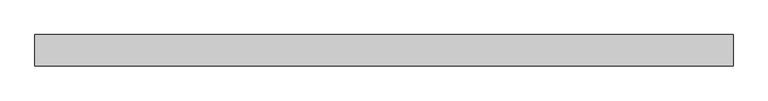
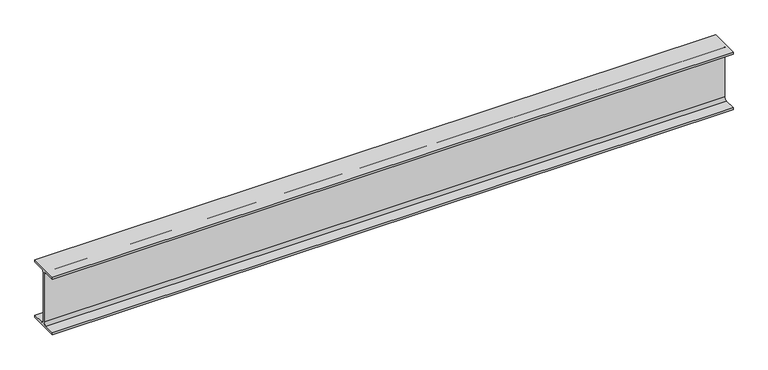
"""IFC4 building model written with IfcOpenShell, lengths in millimetres: beam geometry, 0912_Steel Framing_H-KSD3502 : H_SB_ASB_H-250x125x6x9."""

from ifc_helpers import new_model, si_unit, point, frame, frame_2d, origin, place, context, project, spatial, polyline, circle_curve, trimmed, segment, composite_curve, outline, extrude, source, transform, mapped, element, save


def beam_cbea06df(model_context):
    return source(origin(), model_context, "Body", "SweptSolid", [
        extrude(outline(composite_curve([segment(polyline([(62.5, -116.0), (62.5, -125.0), (-62.5, -125.0), (-62.5, -116.0), (-15.0, -116.0)]), True, "CONTINUOUS"), segment(trimmed(circle_curve(frame_2d((-15.0, -104.0)), 12.0), [point((-15.0, -116.0))], [point((-3.0, -104.0))], True, "CARTESIAN"), True, "CONTINUOUS"), segment(polyline([(-3.0, -104.0), (-3.0, 104.0)]), True, "CONTINUOUS"), segment(trimmed(circle_curve(frame_2d((-15.0, 104.0)), 12.0), [point((-3.0, 104.0))], [point((-15.0, 116.0))], True, "CARTESIAN"), True, "CONTINUOUS"), segment(polyline([(-15.0, 116.0), (-62.5, 116.0), (-62.5, 125.0), (62.5, 125.0), (62.5, 116.0), (15.0, 116.0)]), True, "CONTINUOUS"), segment(trimmed(circle_curve(frame_2d((15.0, 104.0)), 12.0), [point((15.0, 116.0))], [point((3.0, 104.0))], True, "CARTESIAN"), True, "CONTINUOUS"), segment(polyline([(3.0, 104.0), (3.0, -104.0)]), True, "CONTINUOUS"), segment(trimmed(circle_curve(frame_2d((15.0, -104.0)), 12.0), [point((3.0, -104.0))], [point((15.0, -116.0))], True, "CARTESIAN"), True, "CONTINUOUS"), segment(polyline([(15.0, -116.0), (62.5, -116.0)]), True, "CONTINUOUS")], self_intersect=False)), frame((-1382.2982577, 0.0, 0.0), z_axis=(1.0, 0.0, 0.0), x_axis=(0.0, 1.0, 0.0)), (0.0, 0.0, 1.0), 2794.5982507),
    ])


if __name__ == "__main__":
    model = new_model("IFC4")
    model_context = context("Model", 3, world=origin())
    ifc_project = project(units=[si_unit("LENGTHUNIT", "METRE", prefix="MILLI")], contexts=[model_context])
    site = spatial("IfcSite", under=ifc_project)
    building = spatial("IfcBuilding", under=site)
    placement = place(None, origin())
    beam_shape = beam_cbea06df(model_context)
    element("IfcBeam", 1, ObjectType="0912_Steel Framing_H-KSD3502 : H_SB_ASB_H-250x125x6x9", at=placement, inside=building, context=model_context, shape_type="MappedRepresentation", body=[
        mapped(beam_shape, transform((0.0, 0.0, 0.0), x_axis=(1.0, 0.0, 0.0), y_axis=(0.0, 1.0, 0.0), z_axis=(0.0, 0.0, 1.0))),
    ])
    save(model, "model.ifc")

# Revit data of these elements
# Type "0912_Steel Framing_H-KSD3502 : H_SB_ASB_H-250x125x6x9"
#   H_WM Code_1 = "S01AA003-00001 | Main Steel Structure Fabrication Work | Shelter/Building | Light Steel - Standard (30KG/M>Weight) | Material: (   )"
#   H_WM Code_2 = "S03AA029-00001 | Main Steel Structure Erection Work | Shelter/Building | Light Steel (30KG/M>Weight) | Material: (   )"
#   H_WM Code_3 = "S01AA010-00001 | Main Steel Structure Fabrication Work | Shelter/Building | Steel Painting/Coating | for Non-Fireproofed Steel Surface, Surface Preparation, Primer, Second & Final Coat | Material: (   )"
#   H_Q'ty Cal Type Tag = "SB-Q2"
#   Width = 12.5 cm
#   Web Thickness = 0.6 cm
#   Web Fillet = 1.2 cm
#   Warping Constant = 42539.8 cm⁶
#   W = 0
#   Torsional Moment of Inertia = 7.8102 cm⁴
#   Section Area = 37.66 cm²
#   Plastic Modulus weak axis = 73.1 cm³
#   Plastic Modulus strong axis = 366.0 cm³
#   Perimeter = 0.97 m²/m
#   Nominal Weight = 29.60 kgf/m
#   Moment of Inertia weak axis = 294.00 cm⁴
#   Moment of Inertia strong axis = 4050.00 cm⁴
#   Height = 25.0 cm
#   Flange Thickness = 0.9 cm
#   Elastic Modulus weak axis = 47.0 cm³
#   Elastic Modulus strong axis = 324.0 cm³
#   Centroid Vertical = 12.5 cm
#   Centroid Horizontal = 6.25 cm
#   Ix = 40500000
#   Length [instance default] = 1.5240 m
#   Zx = 366000
#   b = 0.1250 m
#   h = 0.2500 m
#   r = 0.0120 m
#   s = 0.0060 m
#   t = 0.0090 m
#   A = 0.003766 m²
#   Structural Material [instance default] = Steel, 45-345
#   Assembly Code = ""
# Element 1 (IfcBeam, "0912_Steel Framing_H-KSD3502 : H_SB_ASB_H-250x125x6x9")
#   Structural Material = none
# Materials
#   "Steel, 45-345": class "Metal", colour RGB 189 187 185, transparency 0, Description = "Steel 345 MPa", Cost = 0
